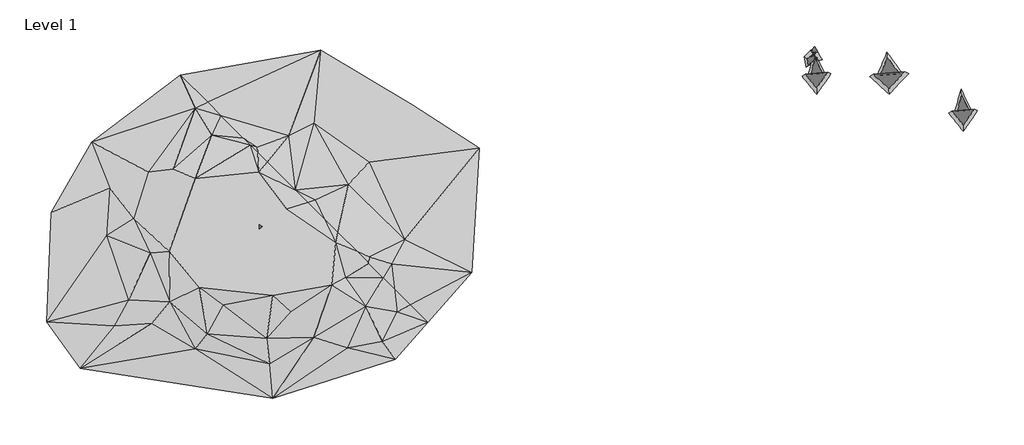
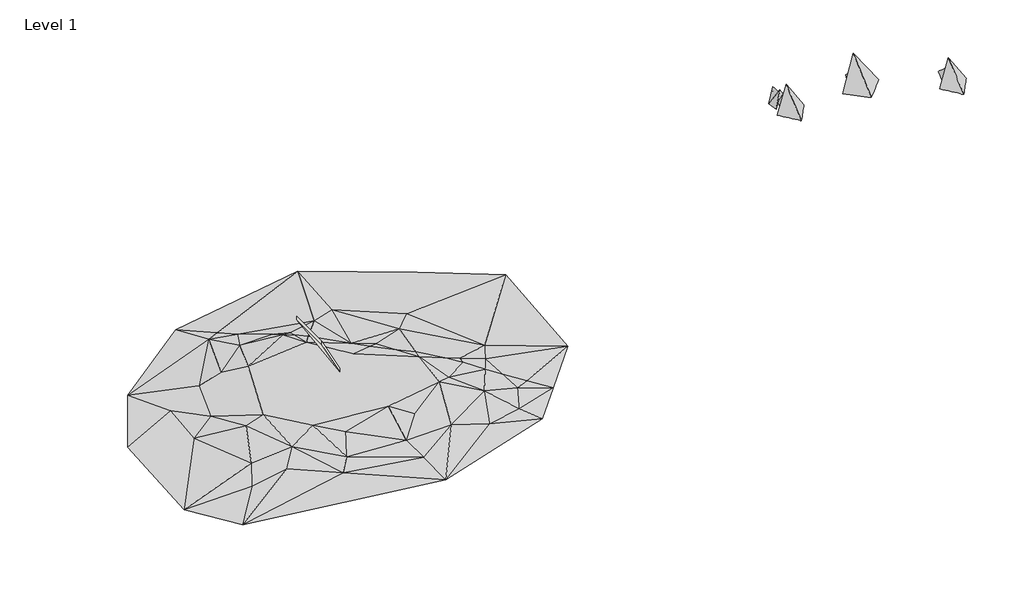
# One storey: 9 proxies, 1 roof.
"""IFC4 building model written with IfcOpenShell, lengths in millimetres."""

import ifcopenshell
import ifcopenshell.guid

model = None  # the IFC model being written
_history = None  # IfcOwnerHistory: only IFC2X3 demands one
_inside = {}  # id of a spatial element -> (the spatial element, [elements in it])
_under = {}  # id of a project, library or spatial element -> (it, [spatial elements below it])
_declared = {}  # id of a project -> (the project, [libraries it declares])
_typed = {}  # id of a type object -> (the type object, [elements of that type])
_made_of = {}  # id of a material, layer set ... -> (it, [elements and type objects made of it])


def new_model(schema):
    """Start an empty IFC model of exactly this schema.

    Asked for "IFC4X3", IfcOpenShell would pick the latest addendum, in which some entities
    have other attributes; the version numbers below select the first issue.
    IFC2X3 requires an IfcOwnerHistory on every rooted entity: one is made here for all.
    """
    global model, _history
    if schema == "IFC4X3":
        model = ifcopenshell.file(schema_version=(4, 3, 0, 0))
    else:
        model = ifcopenshell.file(schema=schema)
    _inside.clear()
    _under.clear()
    _declared.clear()
    _typed.clear()
    _made_of.clear()
    _history = None
    if model.schema == "IFC2X3":
        org = make("IfcOrganization", Name="unknown")
        user = make(
            "IfcPersonAndOrganization",
            ThePerson=make("IfcPerson", FamilyName="unknown"),
            TheOrganization=org,
        )
        app = make(
            "IfcApplication",
            ApplicationDeveloper=org,
            Version="unknown",
            ApplicationFullName="unknown",
            ApplicationIdentifier="unknown",
        )
        _history = make(
            "IfcOwnerHistory",
            OwningUser=user,
            OwningApplication=app,
            ChangeAction="ADDED",
            CreationDate=0,
        )
    return model


def make(cls, **values):
    """One entity of the class cls with the attributes given. An attribute that is None is left unset."""
    return model.create_entity(
        cls, **{name: value for name, value in values.items() if value is not None}
    )


def rooted(cls, **values):
    """An entity with a GlobalId (a new one), such as an element, a storey or a relation."""
    return make(cls, GlobalId=ifcopenshell.guid.new(), OwnerHistory=_history, **values)


def si_unit(unit_type, name, prefix=None):
    """IfcSIUnit, for example si_unit("LENGTHUNIT", "METRE", prefix="MILLI")."""
    return make("IfcSIUnit", UnitType=unit_type, Prefix=prefix, Name=name)


def assignment(units):
    """IfcUnitAssignment: the units of a project."""
    return None if units is None else make("IfcUnitAssignment", Units=units)


def point(xyz):
    """IfcCartesianPoint."""
    return None if xyz is None else make("IfcCartesianPoint", Coordinates=xyz)


def direction(xyz):
    """IfcDirection."""
    return None if xyz is None else make("IfcDirection", DirectionRatios=xyz)


def frame(location, z_axis=None, x_axis=None):
    """IfcAxis2Placement3D, a coordinate frame: its origin and axes. An axis left out is left unset."""
    return make(
        "IfcAxis2Placement3D",
        Location=point(location),
        Axis=direction(z_axis),
        RefDirection=direction(x_axis),
    )


def origin():
    """The frame at (0, 0, 0) with its axes left unset."""
    return frame((0.0, 0.0, 0.0))


def place(relative_to, where):
    """IfcLocalPlacement: puts the frame where relative to a parent placement (None: the world)."""
    return make(
        "IfcLocalPlacement", PlacementRelTo=relative_to, RelativePlacement=where
    )


def context(
    kind, dimensions, precision=None, world=None, true_north=None, identifier=None
):
    """IfcGeometricRepresentationContext, for example the 3D "Model" context."""
    return make(
        "IfcGeometricRepresentationContext",
        ContextIdentifier=identifier,
        ContextType=kind,
        CoordinateSpaceDimension=dimensions,
        Precision=precision,
        WorldCoordinateSystem=world,
        TrueNorth=true_north,
    )


def project(units=None, contexts=None):
    """IfcProject with its units and contexts."""
    return rooted(
        "IfcProject",
        Name="project",
        RepresentationContexts=contexts,
        UnitsInContext=assignment(units),
    )


def spatial(cls, under=None, at=None, **own):
    """A site, building, storey or space (cls), placed at a placement, below another one or the project."""
    s = rooted(cls, ObjectPlacement=at, **own)
    if under is not None:
        _under.setdefault(under.id(), (under, []))[1].append(s)
    return s


def point_list(points):
    """IfcCartesianPointList2D or 3D."""
    cls = (
        "IfcCartesianPointList2D" if len(points[0]) == 2 else "IfcCartesianPointList3D"
    )
    return make(cls, CoordList=points)


def faces_of(points, faces, orient=None, outer=None):
    """IfcFace entities. A face is a list of loops; a loop is a list of indices into points, from 0.

    orient and outer hold one flag for each loop. By default every Orientation is true, the
    first loop of a face is its IfcFaceOuterBound and the others are IfcFaceBound.
    """
    made = []
    for i, loops in enumerate(faces):
        bounds = []
        for j, loop in enumerate(loops):
            is_outer = j == 0 if outer is None else outer[i][j]
            bounds.append(
                make(
                    "IfcFaceOuterBound" if is_outer else "IfcFaceBound",
                    Bound=make("IfcPolyLoop", Polygon=[points[k] for k in loop]),
                    Orientation=True if orient is None else orient[i][j],
                )
            )
        made.append(make("IfcFace", Bounds=bounds))
    return made


def faceted_brep(points, faces, orient=None, outer=None, voids=None):
    """IfcFacetedBrep: a solid bounded by flat faces; with voids (closed shells), ...WithVoids."""
    shared = [point(p) for p in points]
    hull = make("IfcClosedShell", CfsFaces=faces_of(shared, faces, orient, outer))
    if voids is None:
        return make("IfcFacetedBrep", Outer=hull)
    return make(
        "IfcFacetedBrepWithVoids",
        Outer=hull,
        Voids=[
            make(cls, CfsFaces=faces_of(shared, fs, o, b)) for cls, fs, o, b in voids
        ],
    )


def triangles(points, corners, closed=None, point_numbers=None):
    """IfcTriangulatedFaceSet: each triangle names its three corners, points numbered from 1."""
    return make(
        "IfcTriangulatedFaceSet",
        Coordinates=point_list(points),
        Closed=closed,
        CoordIndex=corners,
        PnIndex=point_numbers,
    )


def shape(context_of_items, identifier, shape_type, items):
    """IfcShapeRepresentation: the items that make up one representation, for example the "Body"."""
    return make(
        "IfcShapeRepresentation",
        ContextOfItems=context_of_items,
        RepresentationIdentifier=identifier,
        RepresentationType=shape_type,
        Items=items,
    )


def made_of(thing, what):
    """Note that an element or type object is made of a material, layer set ...; save() writes the relation."""
    if what is not None:
        _made_of.setdefault(what.id(), (what, []))[1].append(thing)
    return thing


def element(
    cls,
    number,
    at=None,
    inside=None,
    cuts=None,
    type_object=None,
    material=None,
    context=None,
    identifier="Body",
    shape_type=None,
    held_by="IfcProductDefinitionShape",
    body=None,
    shapes=None,
    **own,
):
    """One element of the class cls, such as IfcWall. Its Tag is "e" and its number.

    at: its placement. inside: the storey or other place that contains it. cuts: it is an
    opening in that element (IfcRelVoidsElement). A single representation is given by context,
    identifier, shape_type and body (its items); several are given by shapes. held_by: the class
    of the entity that holds the representations. save() writes the other relations.
    """
    e = rooted(cls, Tag="e%d" % number, ObjectPlacement=at, **own)
    if body is not None:
        shapes = [shape(context, identifier, shape_type, body)]
    if shapes is not None:
        e.Representation = make(held_by, Representations=shapes)
    if inside is not None:
        _inside.setdefault(inside.id(), (inside, []))[1].append(e)
    if cuts is not None:
        rooted(
            "IfcRelVoidsElement", RelatingBuildingElement=cuts, RelatedOpeningElement=e
        )
    if type_object is not None:
        _typed.setdefault(type_object.id(), (type_object, []))[1].append(e)
    return made_of(e, material)


def aggregate(whole, parts):
    """IfcRelAggregates: a whole, such as a stair, and the parts it consists of."""
    return rooted("IfcRelAggregates", RelatingObject=whole, RelatedObjects=parts)


def save(model, path):
    """Write the relations noted so far, then the file.

    IfcRelAggregates (storeys below a building ...), IfcRelContainedInSpatialStructure (elements
    in a storey), IfcRelDefinesByType, IfcRelAssociatesMaterial and IfcRelDeclares: one each for
    every whole, place, type object, material and project.
    """
    for whole, parts in _under.values():
        aggregate(whole, parts)
    for where, things in _inside.values():
        rooted(
            "IfcRelContainedInSpatialStructure",
            RelatedElements=things,
            RelatingStructure=where,
        )
    for kind, things in _typed.values():
        rooted("IfcRelDefinesByType", RelatedObjects=things, RelatingType=kind)
    for what, things in _made_of.values():
        rooted("IfcRelAssociatesMaterial", RelatedObjects=things, RelatingMaterial=what)
    for by, libraries in _declared.values():
        rooted("IfcRelDeclares", RelatingContext=by, RelatedDefinitions=libraries)
    model.write(path)


def plane_surface(at):
    """IfcPlane: the flat surface through the origin of the frame at, square to its z axis."""
    return make("IfcPlane", Position=at)


def spline_surface(u_degree, v_degree, points, u_multiplicities, v_multiplicities, u_knots, v_knots, weights=None):
    """IfcBSplineSurfaceWithKnots; with weights, IfcRationalBSplineSurfaceWithKnots. points: one row for each step in u."""
    own = dict(
        UDegree=u_degree,
        VDegree=v_degree,
        ControlPointsList=[[point(p) for p in row] for row in points],
        SurfaceForm="UNSPECIFIED",
        UClosed=False,
        VClosed=False,
        SelfIntersect=False,
        UMultiplicities=u_multiplicities,
        VMultiplicities=v_multiplicities,
        UKnots=u_knots,
        VKnots=v_knots,
        KnotSpec="UNSPECIFIED",
    )
    if weights is None:
        return make("IfcBSplineSurfaceWithKnots", **own)
    return make("IfcRationalBSplineSurfaceWithKnots", WeightsData=weights, **own)


def advanced_brep(points, edges, surfaces, faces):
    """IfcAdvancedBrep: a solid bounded by faces that lie on surfaces and meet in shared edges.

    An edge is (start, end): straight between two places in points (the first is 0);
    or (start, end, curve); or (start, end, curve, False) where it runs against its curve.
    A face is (place in surfaces, loops), or (place, loops, False) where it looks against
    its surface's normal. A loop lists edges by number (the first is 1), with a minus sign
    where the edge is run from its end to its start. The first loop is the outer one.
    """
    corners = [point(p) for p in points]
    vertices = [make("IfcVertexPoint", VertexGeometry=c) for c in corners]
    made = []
    for start, end, *more in edges:
        made.append(
            make(
                "IfcEdgeCurve",
                EdgeStart=vertices[start],
                EdgeEnd=vertices[end],
                EdgeGeometry=more[0] if more else make("IfcPolyline", Points=[corners[start], corners[end]]),
                SameSense=more[1] if len(more) > 1 else True,
            )
        )
    hull = []
    for where, loops, *sense in faces:
        bounds = []
        for j, loop in enumerate(loops):
            ring = [make("IfcOrientedEdge", EdgeElement=made[abs(k) - 1], Orientation=k > 0) for k in loop]
            bounds.append(
                make(
                    "IfcFaceOuterBound" if j == 0 else "IfcFaceBound",
                    Bound=make("IfcEdgeLoop", EdgeList=ring),
                    Orientation=True,
                )
            )
        hull.append(make("IfcAdvancedFace", Bounds=bounds, FaceSurface=surfaces[where], SameSense=sense[0] if sense else True))
    return make("IfcAdvancedBrep", Outer=make("IfcClosedShell", CfsFaces=hull))


model = new_model("IFC4")

# Units and contexts
model_context = context("Model", 3, world=origin())
ifc_project = project(units=[si_unit("LENGTHUNIT", "METRE", prefix="MILLI")], contexts=[model_context])

# Site, building, storey
site = spatial("IfcSite", under=ifc_project)
building = spatial("IfcBuilding", under=site)
storey = spatial("IfcBuildingStorey", under=building, Name="Level 1", Elevation=0.0)

# Proxies
placement = place(None, origin())
element("IfcBuildingElementProxy", 1, Name="Envoltura 3 : Envoltura 3", ObjectType="Envoltura 3 : Envoltura 3", at=placement, inside=storey, context=model_context, shape_type="AdvancedBrep", body=[
    advanced_brep(
    [(149272.8500722, 37183.6261662, 0.0), (145377.1307579, 42480.1094081, 0.0), (145377.1307579, 42480.1094081, 1.0), (145858.2008216, 38691.6629518, 4059.5333521), (143028.7532522, 36708.5635786, 0.0)],
    [
        (0, 1),
        (1, 2),
        (2, 3),
        (3, 0),
        (1, 4),
        (4, 3),
        (4, 0),
    ],
    [
        spline_surface(1, 1, [[(149272.8500722, 37183.6261662, 0.0), (145858.2008216, 38691.6629518, 4059.5333521)], [(145377.1307579, 42480.1094081, 0.0), (145377.1307579, 42480.1094081, 1.0)]], [2, 2], [2, 2], [0.0, 1.0], [0.0, 1.0]),
        spline_surface(1, 1, [[(145377.1307579, 42480.1094081, 0.0), (145377.1307579, 42480.1094081, 1.0)], [(143028.7532522, 36708.5635786, 0.0), (145858.2008216, 38691.6629518, 4059.5333521)]], [2, 2], [2, 2], [0.0, 1.0], [0.0, 1.0]),
        plane_surface(frame((146150.8016622, 36946.0948724, 0.0), z_axis=(0.06958562179180194, -0.9146149815694979, 0.39829295340047827), x_axis=(0.9971182787345019, 0.07586262725179219, 0.0))),
        plane_surface(frame((145892.9113608, 38790.7663843, 0.0), z_axis=(0.0, 0.0, -1.0000000000000002), x_axis=(-0.9971182787345019, -0.07586262725179219, 0.0))),
    ],
    [
        (0, [[1, 2, 3, 4]]),
        (1, [[5, 6, -3, -2]]),
        (2, [[7, -4, -6]]),
        (3, [[-7, -5, -1]]),
    ],
),
])
element("IfcBuildingElementProxy", 2, Name="Envoltura 2 : Envoltura 2", ObjectType="Envoltura 2 : Envoltura 2", at=placement, inside=storey, context=model_context, shape_type="AdvancedBrep", body=[
    advanced_brep(
    [(141557.8692639, 37038.5882122, 0.0), (145882.2043407, 33075.6079455, 0.0), (145882.2043407, 33075.6079455, 1.0), (145651.4124837, 39972.8941629, 6759.3766447), (150238.9901229, 37722.8771323, 0.0)],
    [
        (0, 1),
        (1, 2),
        (2, 3),
        (3, 0),
        (1, 4),
        (4, 3),
        (0, 4),
    ],
    [
        spline_surface(1, 1, [[(141557.8692639, 37038.5882122, 0.0), (145651.4124837, 39972.8941629, 6759.3766447)], [(145882.2043407, 33075.6079455, 0.0), (145882.2043407, 33075.6079455, 1.0)]], [2, 2], [2, 2], [0.0, 1.0], [0.0, 1.0]),
        spline_surface(1, 1, [[(145882.2043407, 33075.6079455, 0.0), (145882.2043407, 33075.6079455, 1.0)], [(150238.9901229, 37722.8771323, 0.0), (145651.4124837, 39972.8941629, 6759.3766447)]], [2, 2], [2, 2], [0.0, 1.0], [0.0, 1.0]),
        plane_surface(frame((145893.0212425, 35945.6910966, 0.0), z_axis=(0.0, 0.0, -1.0), x_axis=(-0.6839386992067904, -0.7295394819523638, 0.0))),
        plane_surface(frame((145898.4296934, 37380.7326722, 0.0), z_axis=(-0.07332961060189151, 0.930284260727444, -0.35943561655986234), x_axis=(-0.9969077163016894, -0.07858120117528421, 0.0))),
    ],
    [
        (0, [[1, 2, 3, 4]]),
        (1, [[5, 6, -3, -2]]),
        (2, [[-5, -1, 7]]),
        (3, [[-7, -4, -6]]),
    ],
),
])
element("IfcBuildingElementProxy", 3, Name="Building Element Proxy", at=placement, inside=storey, context=model_context, shape_type="Tessellation", body=[
    triangles([(-12756.2841614, 37359.2521912, -3983.1676277), (-32583.2506897, 22368.1300232, -3983.1676277), (-41596.3819336, 6600.6593124, -3983.1676277), (-42693.3614868, -17898.520285, -3983.1676277), (-35197.3422913, -28319.8132507, -3983.1676277), (7950.4664566, -35084.511969, -3983.1676277), (35374.9221497, -26308.6871704, -3983.1676277), (42661.7029541, -18058.7372498, -3983.1676277), (38762.9525574, -14159.9833649, -3159.9015999), (35216.0504517, -10613.0824219, -2508.8055862), (32668.7989563, -8065.8320892, -1983.1674671), (29436.9032043, -4833.9340118, -1113.030245), (28710.8893799, -4107.9222221, -983.1675322), (26803.0407166, -2200.0726868, -618.9164371), (22510.7841064, 2092.1850861, -323.039003), (19562.1059509, 5040.8614975, -524.7314521), (15744.845929, 8858.1215195, -714.0854828), (13005.321286, 11597.6467438, -629.5168076), (6704.8674866, 17898.1005432, -542.464018), (4566.221283, 20036.7467468, -763.2442554), (2917.6207489, 21685.3461182, -1136.9525494), (1369.4587063, 23233.5097595, -1431.7908028), (-3672.5964684, 28275.5647888, -2708.6070534), (-6646.9082336, 31249.8762634, -3081.4523186), (-29234.0923279, 1446.318259, -2983.1676201), (-9407.1257996, 29977.8073975, -2983.1676201), (-28508.7156738, 12085.1786133, -2983.1676201), (-27541.5468018, -18864.233432, -2983.1676201), (-9407.1257996, -23941.8711731, -2983.1676201), (7276.5413132, -27326.9622253, -2983.1676201), (24685.5862427, -23700.0789551, -2983.1676201), (35808.0305969, -15720.9334351, -2983.1676201), (32422.9372192, -22249.325647, -2983.1676201), (-5711.4403336, 23898.1389587, -1983.1674671), (-19896.6320435, 15603.4080505, -1983.1674671), (-23142.3967163, 5265.0478134, -1983.1674671), (-24344.5326416, -13007.403717, -1983.1674671), (-19175.351651, -18296.7971375, -1983.1674671), (-6673.1484924, -20580.8530701, -1983.1674671), (6550.3362213, -21662.7754028, -1983.1674671), (17129.1230621, -21422.3482178, -1983.1674671), (28789.8333984, -14449.9656647, -1983.1674671), (-14345.6545898, 16346.8080231, -983.1675322), (-19464.8863037, -2484.6506653, -983.1675322), (-15076.9739044, -13454.4322449, -983.1675322), (-3193.0428909, -14185.7515594, -983.1675322), (11981.8221313, -15648.3890259, -983.1675322), (24231.4116394, -7969.5414551, -983.1675322), (-9409.2529953, 14152.8524048, 16.832463), (-15259.8034424, -2118.9912987, 16.832463), (-8495.1041428, -10163.4982361, 16.832463), (7959.568808, -11991.7947784, 16.832463), (21123.3060059, -9615.0090408, 16.832463), (22037.4548584, -107.8645371, 16.832463), (11067.6732788, 7388.1531052, 16.832463), (4851.4637558, 15615.4898712, 16.832463)], [[4, 5, 28], [28, 5, 38], [4, 28, 37], [25, 37, 44], [37, 25, 4], [36, 44, 50], [44, 36, 25], [37, 45, 44], [25, 36, 27], [28, 38, 37], [4, 25, 3], [45, 38, 29], [29, 38, 5], [39, 29, 30], [45, 29, 39], [50, 45, 51], [50, 44, 45], [49, 50, 55], [51, 45, 39], [39, 46, 51], [50, 51, 55], [39, 40, 46], [45, 37, 38], [5, 6, 29], [36, 50, 49], [25, 27, 3], [49, 43, 36], [36, 35, 27], [3, 27, 2], [1, 2, 26], [35, 2, 27], [2, 35, 26], [43, 26, 35], [36, 43, 35], [43, 49, 34], [34, 49, 21], [34, 21, 22], [26, 24, 1], [24, 26, 23], [34, 23, 26], [23, 34, 22], [26, 43, 34], [20, 21, 56], [56, 21, 49], [51, 46, 52], [41, 30, 6], [30, 40, 39], [31, 6, 7], [41, 6, 31], [55, 51, 52], [52, 40, 47], [41, 53, 47], [41, 47, 40], [40, 30, 41], [47, 53, 52], [42, 41, 31], [30, 29, 6], [33, 7, 8], [7, 33, 31], [33, 8, 32], [42, 53, 41], [10, 42, 32], [32, 9, 10], [9, 32, 8], [42, 33, 32], [33, 42, 31], [11, 42, 10], [16, 55, 54], [56, 49, 55], [55, 52, 54], [55, 16, 17], [56, 19, 20], [19, 56, 18], [18, 56, 55], [55, 17, 18], [52, 53, 54], [48, 11, 12], [48, 53, 42], [48, 12, 13], [54, 15, 16], [15, 54, 14], [14, 54, 48], [48, 13, 14], [48, 54, 53], [42, 11, 48], [52, 46, 40]], closed=False),
])
element("IfcBuildingElementProxy", 4, Name="Building Element Proxy", at=placement, inside=storey, context=model_context, shape_type="Tessellation", body=[
    triangles([(-12757.6003601, 37360.447467, -3983.1676277), (-6648.2244324, 31251.0715393, -3081.4523186), (-3673.9129578, 28276.7600647, -2708.6070534), (1368.1423622, 23234.7050354, -1431.7908028), (2916.3045502, 21686.5437195, -1136.9525494), (4564.9050842, 20037.9420227, -763.2442554), (6703.5512878, 17899.2958191, -542.464018), (13004.0050873, 11598.8420197, -629.5168076), (15743.5297302, 8859.3173767, -714.0854828), (19560.7897522, 5042.0573547, -524.7314521), (22509.4655823, 2093.380798, -323.039003), (26801.7245178, -2198.8769749, -618.9164371), (28709.5731812, -4106.7266556, -983.1675322), (29435.5846802, -4832.7381546, -1113.030245), (32667.4827576, -8064.636232, -1983.1674671), (35214.7342529, -10611.8859833, -2508.8055862), (38761.6363586, -14158.788089, -3159.9015999), (42660.3867554, -18057.5419739, -3983.1676277), (52526.3147827, -6887.5388947, -3983.1676277), (54205.0634766, 21045.4014587, -3983.1676277), (39227.7404663, 30590.2630371, -3983.1676277), (18675.3961212, 42921.6684814, -3983.1676277), (37499.2599243, 480.3448082, -2983.1676201), (29520.1144043, 17889.3882843, -2983.1676201), (17188.7077972, 26593.9116211, -2983.1676201), (34558.7649902, -4951.9041367, -1983.1674671), (24821.4709717, 12839.6930237, -1983.1674671), (11477.7726654, 23779.1206421, -1983.1674671), (29532.1578552, -3397.6033699, -983.1675322), (17465.3967224, 9400.4756241, -983.1675322), (4484.4878998, 21284.4054749, -983.1675322)], [[31, 6, 7], [6, 31, 5], [28, 31, 7], [9, 10, 30], [7, 8, 28], [30, 8, 9], [8, 30, 27], [8, 27, 25], [2, 3, 22], [22, 1, 2], [28, 3, 4], [28, 22, 3], [4, 31, 28], [25, 22, 28], [21, 22, 25], [28, 8, 25], [4, 5, 31], [27, 30, 10], [15, 26, 14], [26, 15, 16], [29, 13, 14], [29, 14, 26], [17, 18, 19], [17, 26, 16], [26, 17, 19], [23, 26, 19], [27, 11, 23], [24, 21, 25], [23, 24, 27], [23, 11, 12], [11, 27, 10], [20, 24, 23], [23, 29, 26], [21, 24, 20], [23, 19, 20], [23, 12, 29], [12, 13, 29], [24, 25, 27]], closed=False),
])
element("IfcBuildingElementProxy", 5, Name="Envoltura 4 : Envoltura 3", ObjectType="Envoltura 4 : Envoltura 3", at=placement, inside=storey, context=model_context, shape_type="AdvancedBrep", body=[
    advanced_brep(
    [(131807.3576386, 37087.3451303, 0.0), (129177.1307579, 42480.1094081, 0.0), (129177.1307579, 42480.1094081, 1.0), (129563.9486784, 38884.9332229, 3300.0), (127620.5407879, 36768.8042581, 0.0)],
    [
        (0, 1),
        (1, 2),
        (2, 3),
        (3, 0),
        (1, 4),
        (4, 3),
        (4, 0),
    ],
    [
        spline_surface(1, 1, [[(131807.3576386, 37087.3451303, 0.0), (129563.9486784, 38884.9332229, 3300.0)], [(129177.1307579, 42480.1094081, 0.0), (129177.1307579, 42480.1094081, 1.0)]], [2, 2], [2, 2], [0.0, 1.0], [0.0, 1.0]),
        spline_surface(1, 1, [[(129177.1307579, 42480.1094081, 0.0), (129177.1307579, 42480.1094081, 1.0)], [(127620.5407879, 36768.8042581, 0.0), (129563.9486784, 38884.9332229, 3300.0)]], [2, 2], [2, 2], [0.0, 1.0], [0.0, 1.0]),
        plane_surface(frame((129713.9492133, 36928.0746942, 0.0), z_axis=(0.0652028601430068, -0.8570091233273167, 0.5111594169756788), x_axis=(0.9971182787345022, 0.07586262725178751, 0.0))),
        plane_surface(frame((129535.0097281, 38778.7529322, 0.0), z_axis=(0.0, 0.0, -1.0), x_axis=(-0.9971182787345022, -0.07586262725178751, 0.0))),
    ],
    [
        (0, [[1, 2, 3, 4]]),
        (1, [[5, 6, -3, -2]]),
        (2, [[7, -4, -6]]),
        (3, [[-7, -5, -1]]),
    ],
),
])
element("IfcBuildingElementProxy", 6, Name="Envoltura 5 : Envoltura 2", ObjectType="Envoltura 5 : Envoltura 2", at=placement, inside=storey, context=model_context, shape_type="AdvancedBrep", body=[
    advanced_brep(
    [(126408.1667764, 37121.3778614, 0.0), (129670.9579301, 33074.7214477, 0.0), (129670.9579301, 33074.7214477, 1.0), (129600.1206686, 39103.6066467, 5300.0), (132851.2952264, 37629.2571411, 0.0)],
    [
        (0, 1),
        (1, 2),
        (2, 3),
        (3, 0),
        (1, 4),
        (4, 3),
        (0, 4),
    ],
    [
        spline_surface(1, 1, [[(126408.1667764, 37121.3778614, 0.0), (129600.1206686, 39103.6066467, 5300.0)], [(129670.9579301, 33074.7214477, 0.0), (129670.9579301, 33074.7214477, 1.0)]], [2, 2], [2, 2], [0.0, 1.0], [0.0, 1.0]),
        spline_surface(1, 1, [[(129670.9579301, 33074.7214477, 0.0), (129670.9579301, 33074.7214477, 1.0)], [(132851.2952264, 37629.2571411, 0.0), (129600.1206686, 39103.6066467, 5300.0)]], [2, 2], [2, 2], [0.0, 1.0], [0.0, 1.0]),
        plane_surface(frame((129643.473311, 35941.7854834, 0.0), z_axis=(0.0, 0.0, -1.0), x_axis=(-0.5725150365089958, -0.8198942205986717, 0.0))),
        plane_surface(frame((129629.7310014, 37375.3175012, 0.0), z_axis=(-0.07472190487376705, 0.9479473771247068, -0.3095357929778475), x_axis=(-0.9969077163016894, -0.07858120117528378, 0.0))),
    ],
    [
        (0, [[1, 2, 3, 4]]),
        (1, [[5, 6, -3, -2]]),
        (2, [[-5, -1, 7]]),
        (3, [[-7, -4, -6]]),
    ],
),
])
element("IfcBuildingElementProxy", 7, Name="Envoltura 6 : Envoltura 1", ObjectType="Envoltura 6 : Envoltura 1", at=placement, inside=storey, context=model_context, shape_type="AdvancedBrep", body=[
    advanced_brep(
    [(129205.8817899, 43770.9712378, 2000.0), (126923.9866586, 41489.0761065, 0.0), (128819.9655331, 40242.3188663, 3500.0), (130887.0468014, 40796.1916228, 1.0), (129205.8817899, 43770.9712378, 0.0), (127302.558064, 39098.8703223, 0.0)],
    [
        (0, 1),
        (1, 2),
        (2, 3),
        (3, 0),
        (3, 4),
        (4, 0),
        (4, 5),
        (5, 1),
        (2, 5),
    ],
    [
        spline_surface(1, 1, [[(126923.9866586, 41489.0761065, 0.0), (129205.8817899, 43770.9712378, 2000.0)], [(128819.9655331, 40242.3188663, 3500.0), (130887.0468014, 40796.1916228, 1.0)]], [2, 2], [2, 2], [0.0, 1.0], [0.0, 1.0]),
        plane_surface(frame((129205.8817899, 43770.9712378, 0.0), z_axis=(0.8705919421583596, 0.49200576241435995, 0.0), x_axis=(-0.4246716312578851, 0.7514458741745219, 0.5049585169009979))),
        spline_surface(1, 1, [[(129205.8817899, 43770.9712378, 0.0), (129205.8817899, 43770.9712378, 2000.0)], [(127302.558064, 39098.8703223, 0.0), (126923.9866586, 41489.0761065, 0.0)]], [2, 2], [2, 2], [0.0, 1.0], [0.0, 1.0]),
        spline_surface(1, 1, [[(127302.558064, 39098.8703223, 0.0), (128819.9655331, 40242.3188663, 3500.0)], [(129205.8817899, 43770.9712378, 0.0), (130887.0468014, 40796.1916228, 1.0)]], [2, 2], [2, 2], [0.0, 1.0], [0.0, 1.0]),
        plane_surface(frame((127302.558064, 39098.8703223, 0.0), z_axis=(-0.8906618919152602, -0.14106698526938924, 0.4322285274677451), x_axis=(0.4545373847315848, -0.2988945620674611, 0.8390815256266055))),
    ],
    [
        (0, [[1, 2, 3, 4]]),
        (1, [[-4, 5, 6]]),
        (2, [[7, 8, -1, -6]]),
        (3, [[-5, -3, 9, -7]]),
        (4, [[-2, -8, -9]]),
    ],
),
])
element("IfcBuildingElementProxy", 8, Name="Envoltura 7 : Envoltura 3", ObjectType="Envoltura 7 : Envoltura 3", at=placement, inside=storey, context=model_context, shape_type="AdvancedBrep", body=[
    advanced_brep(
    [(164616.9519856, 28819.6206164, 0.0), (161986.7251048, 34212.3848942, 0.0), (161986.7251048, 34212.3848942, 1.0), (162373.5430253, 30617.208709, 3300.0), (160430.1351349, 28501.0797442, 0.0)],
    [
        (0, 1),
        (1, 2),
        (2, 3),
        (3, 0),
        (1, 4),
        (4, 3),
        (4, 0),
    ],
    [
        spline_surface(1, 1, [[(164616.9519856, 28819.6206164, 0.0), (162373.5430253, 30617.208709, 3300.0)], [(161986.7251048, 34212.3848942, 0.0), (161986.7251048, 34212.3848942, 1.0)]], [2, 2], [2, 2], [0.0, 1.0], [0.0, 1.0]),
        spline_surface(1, 1, [[(161986.7251048, 34212.3848942, 0.0), (161986.7251048, 34212.3848942, 1.0)], [(160430.1351349, 28501.0797442, 0.0), (162373.5430253, 30617.208709, 3300.0)]], [2, 2], [2, 2], [0.0, 1.0], [0.0, 1.0]),
        plane_surface(frame((162523.5435602, 28660.3501803, 0.0), z_axis=(0.0652028601430068, -0.8570091233273167, 0.5111594169756788), x_axis=(0.9971182787345022, 0.07586262725178751, 0.0))),
        plane_surface(frame((162344.6040751, 30511.0284182, 0.0), z_axis=(0.0, 0.0, -1.0), x_axis=(-0.9971182787345022, -0.07586262725178751, 0.0))),
    ],
    [
        (0, [[1, 2, 3, 4]]),
        (1, [[5, 6, -3, -2]]),
        (2, [[7, -4, -6]]),
        (3, [[-7, -5, -1]]),
    ],
),
])
element("IfcBuildingElementProxy", 9, Name="Envoltura 8 : Envoltura 2", ObjectType="Envoltura 8 : Envoltura 2", at=placement, inside=storey, context=model_context, shape_type="AdvancedBrep", body=[
    advanced_brep(
    [(159217.7611234, 28853.6533475, 0.0), (162480.5522771, 24806.9969338, 0.0), (162480.5522771, 24806.9969338, 1.0), (162409.7150156, 30835.8821327, 5300.0), (165660.8895734, 29361.5326272, 0.0)],
    [
        (0, 1),
        (1, 2),
        (2, 3),
        (3, 0),
        (1, 4),
        (4, 3),
        (0, 4),
    ],
    [
        spline_surface(1, 1, [[(159217.7611234, 28853.6533475, 0.0), (162409.7150156, 30835.8821327, 5300.0)], [(162480.5522771, 24806.9969338, 0.0), (162480.5522771, 24806.9969338, 1.0)]], [2, 2], [2, 2], [0.0, 1.0], [0.0, 1.0]),
        spline_surface(1, 1, [[(162480.5522771, 24806.9969338, 0.0), (162480.5522771, 24806.9969338, 1.0)], [(165660.8895734, 29361.5326272, 0.0), (162409.7150156, 30835.8821327, 5300.0)]], [2, 2], [2, 2], [0.0, 1.0], [0.0, 1.0]),
        plane_surface(frame((162453.067658, 27674.0609695, 0.0), z_axis=(0.0, 0.0, -1.0), x_axis=(-0.5725150365089958, -0.8198942205986717, 0.0))),
        plane_surface(frame((162439.3253484, 29107.5929873, 0.0), z_axis=(-0.07472190487376705, 0.9479473771247068, -0.3095357929778475), x_axis=(-0.9969077163016894, -0.07858120117528378, 0.0))),
    ],
    [
        (0, [[1, 2, 3, 4]]),
        (1, [[5, 6, -3, -2]]),
        (2, [[-5, -1, 7]]),
        (3, [[-7, -4, -6]]),
    ],
),
])

# Roof
element("IfcRoof", 10, ObjectType="Generic - 400mm", at=placement, inside=storey, context=model_context, shape_type="Brep", body=[
    faceted_brep([(-1448.0641066, -1617.3453083, 12124.355653), (-1448.0641066, 8382.6546917, 12124.355653), (5551.9358934, 3382.6546917, 0.0), (-1448.0641066, 8382.6546917, 12924.355653), (-1448.0641066, -1617.3453083, 12924.355653), (5551.9358934, 3382.6546917, 800.0)], [[[0, 1, 2]], [[3, 4, 5]], [[4, 3, 1, 0]], [[5, 4, 0, 2]], [[3, 5, 2, 1]]]),
])

save(model, "model.ifc")

# Revit data of these elements
# Project information
#   Project Issue Date = "Issue Date"
#   Project Status = "Project Status"
#   Client Name = "Owner"
#   Project Address = "Enter address here"
#   Project Name = "Project Name"
#   Project Number = "0001"
# Type "Generic - 400mm"
#   Layers, outside or top first: 0.40 m no material (function 1)
# Element 1 (IfcBuildingElementProxy, "Envoltura 3 : Envoltura 3")
#   Phase Created = New Construction
#   Materials on its faces: "Default Form"
# Element 2 (IfcBuildingElementProxy, "Envoltura 2 : Envoltura 2")
#   Phase Created = New Construction
#   Materials on its faces: "Default Form"
# Elements 3, 4 (IfcBuildingElementProxy)
#   Material = none
#   Phase Created = New Construction
# Element 5 (IfcBuildingElementProxy, "Envoltura 4 : Envoltura 3")
#   Phase Created = New Construction
#   Materials on its faces: "Default Form"
# Element 6 (IfcBuildingElementProxy, "Envoltura 5 : Envoltura 2")
#   Phase Created = New Construction
#   Materials on its faces: "Default Form"
# Element 7 (IfcBuildingElementProxy, "Envoltura 6 : Envoltura 1")
#   Phase Created = New Construction
#   Materials on its faces: "Default Form"
# Element 8 (IfcBuildingElementProxy, "Envoltura 7 : Envoltura 3")
#   Phase Created = New Construction
#   Materials on its faces: "Default Form"
# Element 9 (IfcBuildingElementProxy, "Envoltura 8 : Envoltura 2")
#   Phase Created = New Construction
#   Materials on its faces: "Default Form"
# Element 10 (IfcRoof, "Generic - 400mm")
#   built-in parameter 1001705 = 42.4027 (stored number, unit not read)
#   built-in parameter 1001710 = 33615
#   Phase Created = New Construction
#   Materials on its faces: "Default Roof"
# Materials
#   "Default Form": class "Generic", colour RGB 185 189 196, transparency 0.5, Cost = 0
#   "Default Roof": class "Miscellaneous", colour RGB 0 127 0, transparency 0, Cost = 0
